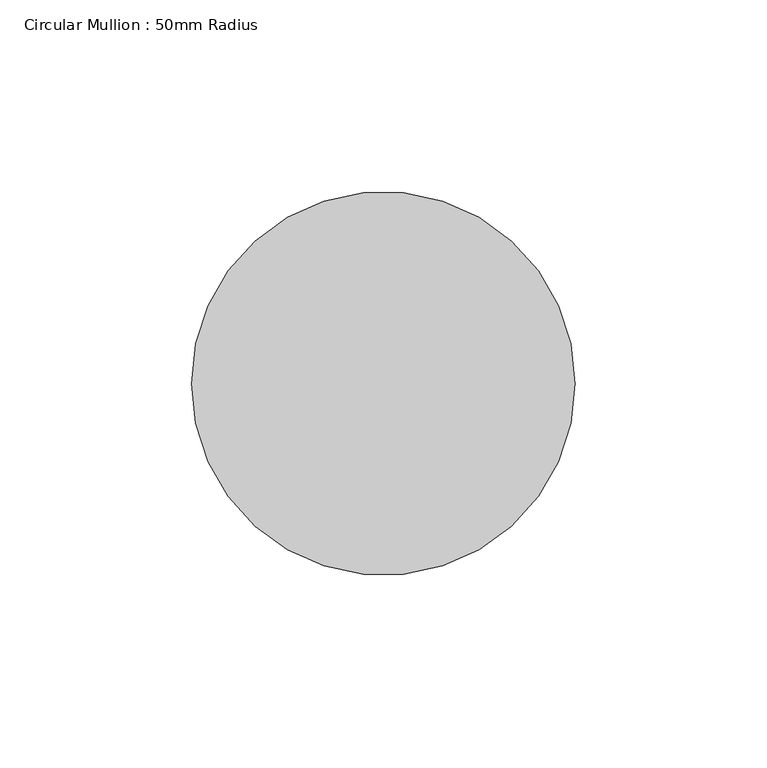
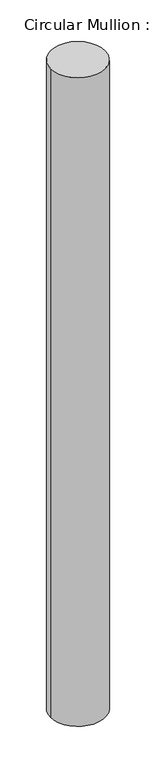
"""IFC4 building model written with IfcOpenShell, lengths in millimetres: member geometry, Circular Mullion : 50mm Radius."""

from ifc_helpers import new_model, si_unit, point, frame, origin, origin_2d, place, context, project, spatial, circle_curve, trimmed, segment, composite_curve, outline, extrude, source, transform, mapped, element, save


def circular_mullion_50mm_radius_1284f4c3(model_context):
    return source(origin(), model_context, "Body", "SweptSolid", [
        extrude(outline(composite_curve([segment(trimmed(circle_curve(origin_2d(), 50.0), [point((50.0, 0.0))], [point((-50.0, 0.0))], False, "CARTESIAN"), True, "CONTINUOUS"), segment(trimmed(circle_curve(origin_2d(), 50.0), [point((-50.0, 0.0))], [point((50.0, 0.0))], False, "CARTESIAN"), True, "CONTINUOUS")], self_intersect=False)), frame((0.0, 0.0, -1253.2485873), z_axis=(0.0, 0.0, 1.0), x_axis=(1.0, 0.0, 0.0)), (0.0, 0.0, 1.0), 1253.2485873),
    ])


if __name__ == "__main__":
    model = new_model("IFC4")
    model_context = context("Model", 3, world=origin())
    ifc_project = project(units=[si_unit("LENGTHUNIT", "METRE", prefix="MILLI")], contexts=[model_context])
    site = spatial("IfcSite", under=ifc_project)
    building = spatial("IfcBuilding", under=site)
    placement = place(None, origin())
    circular_mullion_50mm_radius_shape = circular_mullion_50mm_radius_1284f4c3(model_context)
    element("IfcMember", 1, ObjectType="Circular Mullion : 50mm Radius", at=placement, inside=building, context=model_context, shape_type="MappedRepresentation", body=[
        mapped(circular_mullion_50mm_radius_shape, transform((0.0, 0.0, 0.0), x_axis=(1.0, 0.0, 0.0), y_axis=(0.0, 1.0, 0.0), z_axis=(0.0, 0.0, 1.0))),
    ])
    save(model, "model.ifc")

# Revit data of these elements
# Type "Circular Mullion : 50mm Radius"
#   built-in parameter 1007350 = 0.164042 (stored number, unit not read)
# Element 1 (IfcMember, "Circular Mullion : 50mm Radius")
#   Materials on its faces: "Aluminium"
# Materials
#   "Aluminium": class "Metal", colour RGB 247 247 247, transparency 0, Description = "Aluminium 6061", Cost = 0
